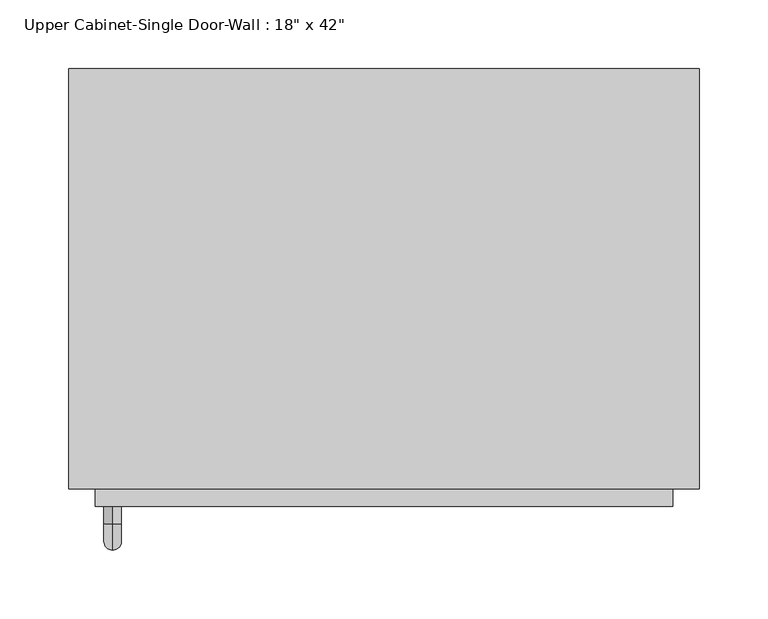
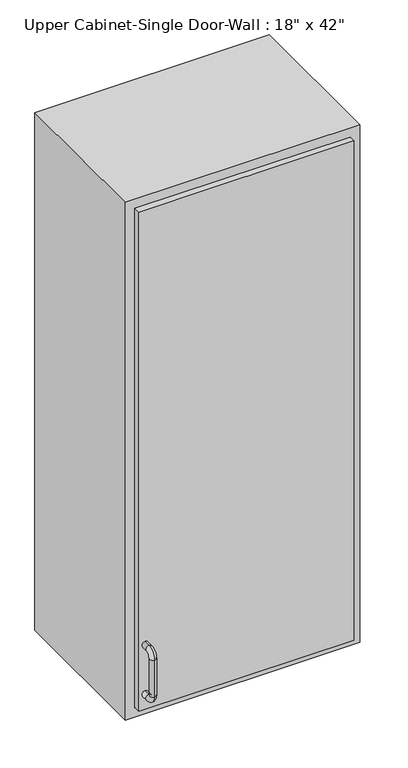
"""IFC4 building model written with IfcOpenShell, lengths in millimetres: furniture geometry."""

from ifc_helpers import new_model, si_unit, point, frame, origin, place, context, project, spatial, polyline, circle_curve, ellipse_curve, trimmed, outline, extrude, faceted_brep, source, transform, mapped, element, save
from ifc_brep_helpers import plane_surface, cylinder_surface, revolved_surface, advanced_brep


def furniture_53c638ad(model_context):
    return source(origin(), model_context, "Body", "SolidModel", [
        faceted_brep([(-198.8288372, -61.9125, 2438.4), (258.3711628, -61.9125, 2438.4), (258.3711628, -61.9125, 1371.6), (-198.8288372, -61.9125, 1371.6), (-198.8288372, -366.7125, 2438.4), (-198.8288372, -366.7125, 1371.6), (258.3711628, -366.7125, 1371.6), (258.3711628, -366.7125, 2438.4), (-179.7788372, -366.7125, 2419.35), (239.3211628, -366.7125, 2419.35), (239.3211628, -366.7125, 1390.65), (-179.7788372, -366.7125, 1390.65), (-179.7788372, -80.9625, 2419.35), (239.3211628, -80.9625, 2419.35), (239.3211628, -80.9625, 1390.65), (-179.7788372, -80.9625, 1390.65)], [[[0, 1, 2, 3]], [[4, 5, 6, 7], [8, 9, 10, 11]], [[3, 5, 4, 0]], [[2, 6, 5, 3]], [[1, 7, 6, 2]], [[0, 4, 7, 1]], [[8, 12, 13, 9]], [[9, 13, 14, 10]], [[10, 14, 15, 11]], [[11, 15, 12, 8]], [[12, 15, 14, 13]]]),
        advanced_brep(
        [(-167.0788372, -379.4125, 1517.65), (-167.0788372, -379.4125, 1530.35), (-167.0788372, -392.1125, 1530.35), (-167.0788372, -392.1125, 1517.65), (-167.0788372, -411.1625, 1511.3), (-167.0788372, -398.4625, 1511.3), (-167.0788372, -411.1625, 1435.1), (-167.0788372, -398.4625, 1435.1), (-167.0788372, -392.1125, 1416.05), (-167.0788372, -392.1125, 1428.75), (-167.0788372, -379.4125, 1428.75), (-167.0788372, -379.4125, 1416.05)],
        [
            (0, 1, circle_curve(frame((-167.0788372, -379.4125, 1524.0), z_axis=(0.0, 1.0, 0.0), x_axis=(0.0, 0.0, 1.0)), 6.35)),
            (1, 0, circle_curve(frame((-167.0788372, -379.4125, 1524.0), z_axis=(0.0, 1.0, 0.0), x_axis=(0.0, 0.0, 1.0)), 6.35)),
            (1, 2),
            (2, 3, circle_curve(frame((-167.0788372, -392.1125, 1524.0), z_axis=(0.0, 1.0, 0.0), x_axis=(0.0, 0.0, 1.0)), 6.35)),
            (3, 0),
            (3, 2, circle_curve(frame((-167.0788372, -392.1125, 1524.0), z_axis=(0.0, 1.0, 0.0), x_axis=(0.0, 0.0, 1.0)), 6.35)),
            (4, 5, circle_curve(frame((-167.0788372, -404.8125, 1511.3), z_axis=(0.0, 0.0, 1.0), x_axis=(0.0, -1.0, 0.0)), 6.35)),
            (5, 3, circle_curve(frame((-167.0788372, -392.1125, 1511.3), z_axis=(-1.0, 0.0, 0.0), x_axis=(0.0, 0.0, 1.0)), 6.35)),
            (2, 4, circle_curve(frame((-167.0788372, -392.1125, 1511.3), z_axis=(1.0, 0.0, 0.0), x_axis=(0.0, 0.0, 1.0)), 19.05)),
            (5, 4, circle_curve(frame((-167.0788372, -404.8125, 1511.3), z_axis=(0.0, 0.0, 1.0), x_axis=(0.0, -1.0, 0.0)), 6.35)),
            (4, 6),
            (6, 7, circle_curve(frame((-167.0788372, -404.8125, 1435.1), z_axis=(0.0, 0.0, 1.0), x_axis=(0.0, -1.0, 0.0)), 6.35)),
            (7, 5),
            (7, 6, circle_curve(frame((-167.0788372, -404.8125, 1435.1), z_axis=(0.0, 0.0, 1.0), x_axis=(0.0, -1.0, 0.0)), 6.35)),
            (8, 9, circle_curve(frame((-167.0788372, -392.1125, 1422.4), z_axis=(0.0, -1.0, 0.0), x_axis=(0.0, 0.0, -1.0)), 6.35)),
            (9, 7, circle_curve(frame((-167.0788372, -392.1125, 1435.1), z_axis=(-1.0, 0.0, 0.0), x_axis=(0.0, -1.0, 0.0)), 6.35)),
            (6, 8, circle_curve(frame((-167.0788372, -392.1125, 1435.1), z_axis=(1.0, 0.0, 0.0), x_axis=(0.0, -1.0, 0.0)), 19.05)),
            (9, 8, circle_curve(frame((-167.0788372, -392.1125, 1422.4), z_axis=(0.0, -1.0, 0.0), x_axis=(0.0, 0.0, -1.0)), 6.35)),
            (10, 11, circle_curve(frame((-167.0788372, -379.4125, 1422.4), z_axis=(0.0, 1.0, 0.0), x_axis=(0.0, 0.0, -1.0)), 6.35)),
            (11, 10, circle_curve(frame((-167.0788372, -379.4125, 1422.4), z_axis=(0.0, 1.0, 0.0), x_axis=(0.0, 0.0, -1.0)), 6.35)),
            (8, 11),
            (10, 9),
        ],
        [
            plane_surface(frame((-173.4288372, -379.4125, 1524.0), z_axis=(0.0, 1.0, 0.0), x_axis=(0.0, 0.0, 1.0))),
            cylinder_surface(frame((-167.0788372, -379.4125, 1524.0), z_axis=(0.0, 1.0, 0.0), x_axis=(0.0, 0.0, 1.0)), 6.35),
            revolved_surface(trimmed(ellipse_curve(frame((-167.0788372, -392.1125, 1524.0), z_axis=(0.0, -1.0, 0.0), x_axis=(0.0, 0.0, 1.0)), 6.35, 6.35), [point((-167.0788372, -392.1125, 1517.65))], [point((-167.0788372, -392.1125, 1530.35))], True, "CARTESIAN"), (-167.0788372, -392.1125, 1511.3), (-1.0, 0.0, 0.0)),
            revolved_surface(trimmed(ellipse_curve(frame((-167.0788372, -392.1125, 1524.0), z_axis=(0.0, -1.0, 0.0), x_axis=(0.0, 0.0, 1.0)), 6.35, 6.35), [point((-167.0788372, -392.1125, 1530.35))], [point((-167.0788372, -392.1125, 1517.65))], True, "CARTESIAN"), (-167.0788372, -392.1125, 1511.3), (-1.0, 0.0, 0.0)),
            cylinder_surface(frame((-167.0788372, -404.8125, 1511.3), z_axis=(0.0, 0.0, 1.0), x_axis=(0.0, -1.0, 0.0)), 6.35),
            revolved_surface(trimmed(ellipse_curve(frame((-167.0788372, -404.8125, 1435.1), z_axis=(0.0, 0.0, -1.0), x_axis=(0.0, -1.0, 0.0)), 6.35, 6.35), [point((-167.0788372, -398.4625, 1435.1))], [point((-167.0788372, -411.1625, 1435.1))], True, "CARTESIAN"), (-167.0788372, -392.1125, 1435.1), (-1.0, 0.0, 0.0)),
            revolved_surface(trimmed(ellipse_curve(frame((-167.0788372, -404.8125, 1435.1), z_axis=(0.0, 0.0, -1.0), x_axis=(0.0, -1.0, 0.0)), 6.35, 6.35), [point((-167.0788372, -411.1625, 1435.1))], [point((-167.0788372, -398.4625, 1435.1))], True, "CARTESIAN"), (-167.0788372, -392.1125, 1435.1), (-1.0, 0.0, 0.0)),
            plane_surface(frame((-173.4288372, -379.4125, 1422.4), z_axis=(0.0, 1.0, 0.0), x_axis=(0.0, 0.0, -1.0))),
            cylinder_surface(frame((-167.0788372, -392.1125, 1422.4), z_axis=(0.0, -1.0, 0.0), x_axis=(0.0, 0.0, -1.0)), 6.35),
        ],
        [
            (0, [[1, 2]]),
            (1, [[3, 4, 5, -2]]),
            (1, [[-5, 6, -3, -1]]),
            (2, [[7, 8, -4, 9]]),
            (3, [[10, -9, -6, -8]]),
            (4, [[11, 12, 13, -7]]),
            (4, [[-13, 14, -11, -10]]),
            (5, [[15, 16, -12, 17]]),
            (6, [[18, -17, -14, -16]]),
            (7, [[19, 20]]),
            (8, [[21, -19, 22, -15]]),
            (8, [[-22, -20, -21, -18]]),
        ],
    ),
        extrude(outline(polyline([(-179.7788372, -379.4125), (-179.7788372, -347.6625), (239.3211628, -347.6625), (239.3211628, -379.4125), (-179.7788372, -379.4125)])), frame((0.0, 0.0, 1390.65), z_axis=(0.0, 0.0, 1.0), x_axis=(1.0, 0.0, 0.0)), (0.0, 0.0, 1.0), 1028.7),
    ])


if __name__ == "__main__":
    model = new_model("IFC4")
    model_context = context("Model", 3, world=origin())
    ifc_project = project(units=[si_unit("LENGTHUNIT", "METRE", prefix="MILLI")], contexts=[model_context])
    site = spatial("IfcSite", under=ifc_project)
    building = spatial("IfcBuilding", under=site)
    placement = place(None, origin())
    furniture_shape = furniture_53c638ad(model_context)
    element("IfcFurniture", 1, ObjectType="Upper Cabinet-Single Door-Wall : 18\" x 42\"", at=placement, inside=building, context=model_context, shape_type="MappedRepresentation", body=[
        mapped(furniture_shape, transform((0.0, 0.0, 0.0), x_axis=(1.0, 0.0, 0.0), y_axis=(0.0, 1.0, 0.0), z_axis=(0.0, 0.0, 1.0))),
    ])
    save(model, "model.ifc")

# Revit data of these elements
# Type "Upper Cabinet-Single Door-Wall : 18\" x 42\""
#   COBie.Type.CreatedBy = "doug.wood@us.ibm.com"
#   COBie.Type.CreatedOn = "2016-04-14T02:07:23"
#   COBie.Type.Name = "Casework_Upper Cabinet-Single Door-Wall_18\" x 42\""
#   COBie.Type.Category = "23-40 35 17 47 11 : Kitchen Casework"
#   COBie.Type.Description = "Upper Cabinet-Single Door-Wall_18\" x 42\""
#   COBie.Type.Manufacturer = ""
#   COBie.Type.ModelNumber = ""
#   Assembly Code = "C1030410"
#   COBie.Type.ReplacementCost = 0
#   Depth = 1' - 0"
#   Height = 3' - 6"
#   Top Of Cabinet = 8' - 0"
#   Width = 1' - 6"
#   COBie.Type = no
#   Cabinet Material = none
#   Door/Drawer Material = none
#   Handle Material = Cabinets - Handles
# Element 1 (IfcFurniture, "Upper Cabinet-Single Door-Wall : 18\" x 42\"")
#   Materials on its faces: "Cabinets", "Cabinets - Handles"
# Materials
#   "Cabinets - Handles": class "Metal", colour RGB 57 57 57, transparency 0
#   "Cabinets": class "Miscellaneous", colour RGB 249 249 249, transparency 0
